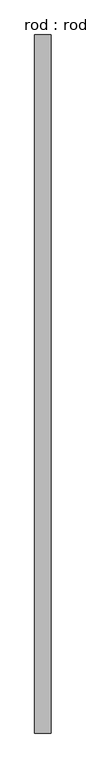
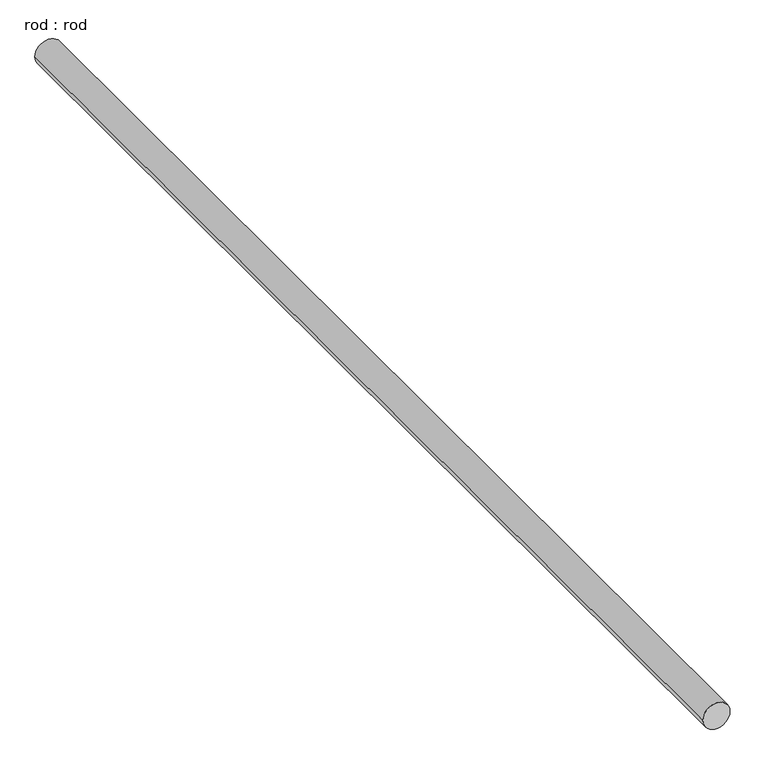
"""IFC4 building model written with IfcOpenShell, lengths in millimetres: proxy geometry, rod : rod."""

from ifc_helpers import new_model, si_unit, point, frame, frame_2d, origin, place, context, project, spatial, circle_curve, trimmed, segment, composite_curve, outline, extrude, source, transform, mapped, element, save


def rod_rod_666800db(model_context):
    return source(origin(), model_context, "Body", "SweptSolid", [
        extrude(outline(composite_curve([segment(trimmed(circle_curve(frame_2d((0.0108462, 0.0)), 200.0), [point((0.0108462, 200.0))], [point((0.0108462, -200.0))], False, "CARTESIAN"), True, "CONTINUOUS"), segment(trimmed(circle_curve(frame_2d((0.0108462, 0.0)), 200.0), [point((0.0108462, -200.0))], [point((0.0108462, 200.0))], False, "CARTESIAN"), True, "CONTINUOUS")], self_intersect=False)), frame((0.0, -4449.4324476, 0.0), z_axis=(0.0, 1.0, 0.0), x_axis=(0.0, 0.0, 1.0)), (0.0, 0.0, 1.0), 17084.3221259),
    ])


if __name__ == "__main__":
    model = new_model("IFC4")
    model_context = context("Model", 3, world=origin())
    ifc_project = project(units=[si_unit("LENGTHUNIT", "METRE", prefix="MILLI")], contexts=[model_context])
    site = spatial("IfcSite", under=ifc_project)
    building = spatial("IfcBuilding", under=site)
    placement = place(None, origin())
    rod_rod_shape = rod_rod_666800db(model_context)
    element("IfcBuildingElementProxy", 1, Name="rod : rod", ObjectType="rod : rod", at=placement, inside=building, context=model_context, shape_type="MappedRepresentation", body=[
        mapped(rod_rod_shape, transform((0.0, 0.0, 0.0), x_axis=(1.0, 0.0, 0.0), y_axis=(0.0, 1.0, 0.0), z_axis=(0.0, 0.0, 1.0))),
    ])
    save(model, "model.ifc")

# Revit data of these elements
# Type "rod : rod"
#   Default Elevation = 0
